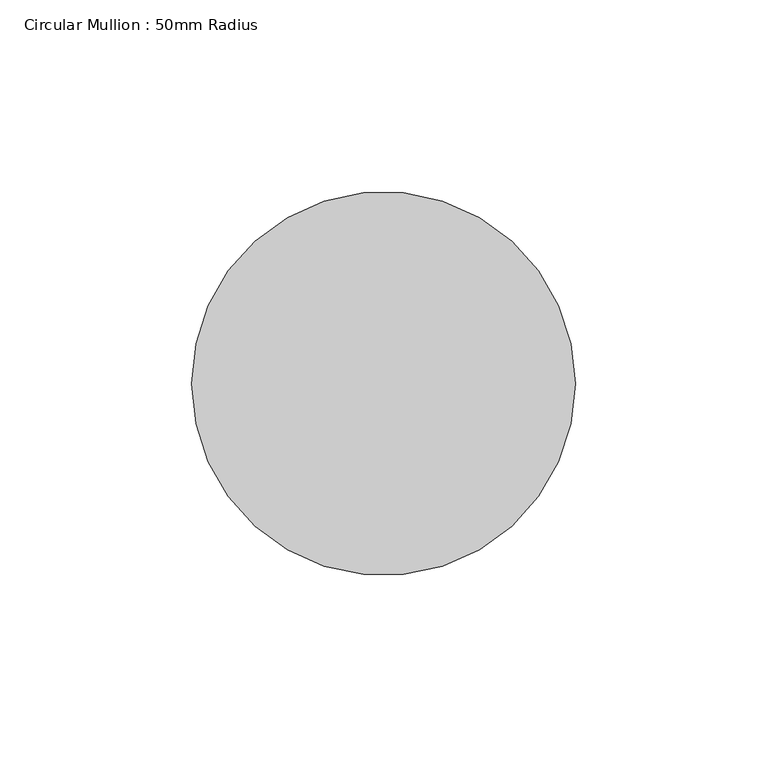
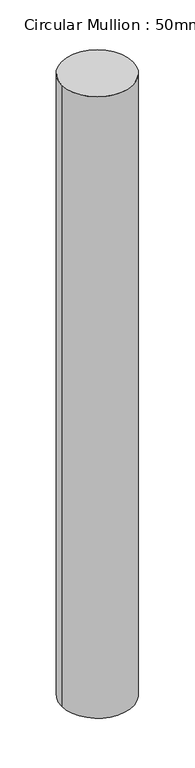
"""IFC4 building model written with IfcOpenShell, lengths in millimetres: member geometry, Circular Mullion : 50mm Radius."""

from ifc_helpers import new_model, si_unit, point, frame, origin, origin_2d, place, context, project, spatial, circle_curve, trimmed, segment, composite_curve, outline, extrude, source, transform, mapped, element, save


def circular_mullion_50mm_radius_a04fa95b(model_context):
    return source(origin(), model_context, "Body", "SweptSolid", [
        extrude(outline(composite_curve([segment(trimmed(circle_curve(origin_2d(), 50.0), [point((50.0, 0.0))], [point((-50.0, 0.0))], False, "CARTESIAN"), True, "CONTINUOUS"), segment(trimmed(circle_curve(origin_2d(), 50.0), [point((-50.0, 0.0))], [point((50.0, 0.0))], False, "CARTESIAN"), True, "CONTINUOUS")], self_intersect=False)), frame((0.0, 0.0, -922.5604929), z_axis=(0.0, 0.0, 1.0), x_axis=(1.0, 0.0, 0.0)), (0.0, 0.0, 1.0), 922.5604929),
    ])


if __name__ == "__main__":
    model = new_model("IFC4")
    model_context = context("Model", 3, world=origin())
    ifc_project = project(units=[si_unit("LENGTHUNIT", "METRE", prefix="MILLI")], contexts=[model_context])
    site = spatial("IfcSite", under=ifc_project)
    building = spatial("IfcBuilding", under=site)
    placement = place(None, origin())
    circular_mullion_50mm_radius_shape = circular_mullion_50mm_radius_a04fa95b(model_context)
    element("IfcMember", 1, ObjectType="Circular Mullion : 50mm Radius", at=placement, inside=building, context=model_context, shape_type="MappedRepresentation", body=[
        mapped(circular_mullion_50mm_radius_shape, transform((0.0, 0.0, 0.0), x_axis=(1.0, 0.0, 0.0), y_axis=(0.0, 1.0, 0.0), z_axis=(0.0, 0.0, 1.0))),
    ])
    save(model, "model.ifc")

# Revit data of these elements
# Type "Circular Mullion : 50mm Radius"
#   built-in parameter 1007350 = 0.164042 (stored number, unit not read)
# Element 1 (IfcMember, "Circular Mullion : 50mm Radius")
#   Materials on its faces: "Aluminium"
# Materials
#   "Aluminium": class "Metal", colour RGB 247 247 247, transparency 0, Description = "Aluminium 6061", Cost = 0
